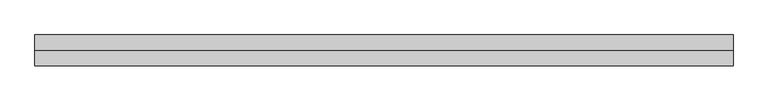
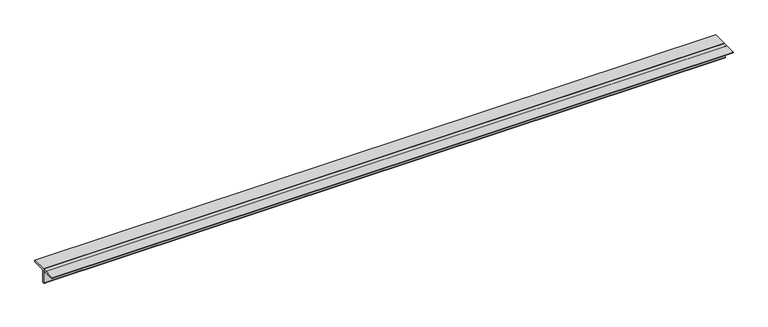
"""IFC4 building model written with IfcOpenShell, lengths in millimetres: member geometry, Steel Framing_2Ls_KS : H_SB_AR_S02_2Ls-100x100x10_VBR1."""

from ifc_helpers import new_model, si_unit, point, frame, frame_2d, origin, place, context, project, spatial, polyline, circle_curve, trimmed, segment, composite_curve, outline, extrude, source, transform, mapped, element, save


def member_d81a11a3(model_context):
    return source(origin(), model_context, "Body", "SweptSolid", [
        extrude(outline(composite_curve([segment(polyline([(0.0, 28.2), (100.0, 28.2)]), True, "CONTINUOUS"), segment(trimmed(circle_curve(frame_2d((90.0, 28.2)), 10.0), [point((100.0, 28.2))], [point((90.0, 18.2))], False, "CARTESIAN"), True, "CONTINUOUS"), segment(polyline([(90.0, 18.2), (20.0, 18.2)]), True, "CONTINUOUS"), segment(trimmed(circle_curve(frame_2d((20.0, 8.2)), 10.0), [point((20.0, 18.2))], [point((10.0, 8.2))], True, "CARTESIAN"), True, "CONTINUOUS"), segment(polyline([(10.0, 8.2), (10.0, -61.8)]), True, "CONTINUOUS"), segment(trimmed(circle_curve(frame_2d((0.0, -61.8)), 10.0), [point((10.0, -61.8))], [point((0.0, -71.8))], False, "CARTESIAN"), True, "CONTINUOUS"), segment(polyline([(0.0, -71.8), (0.0, 28.2)]), True, "CONTINUOUS")], self_intersect=False)), frame((-2072.1213123, 0.0, 0.0), z_axis=(1.0, 0.0, 0.0), x_axis=(0.0, 1.0, 0.0)), (0.0, 0.0, 1.0), 4551.278999),
        extrude(outline(composite_curve([segment(polyline([(0.0, 28.2), (0.0, -71.8)]), True, "CONTINUOUS"), segment(trimmed(circle_curve(frame_2d((0.0, -61.8)), 10.0), [point((0.0, -71.8))], [point((-10.0, -61.8))], False, "CARTESIAN"), True, "CONTINUOUS"), segment(polyline([(-10.0, -61.8), (-10.0, 8.2)]), True, "CONTINUOUS"), segment(trimmed(circle_curve(frame_2d((-20.0, 8.2)), 10.0), [point((-10.0, 8.2))], [point((-20.0, 18.2))], True, "CARTESIAN"), True, "CONTINUOUS"), segment(polyline([(-20.0, 18.2), (-90.0, 18.2)]), True, "CONTINUOUS"), segment(trimmed(circle_curve(frame_2d((-90.0, 28.2)), 10.0), [point((-90.0, 18.2))], [point((-100.0, 28.2))], False, "CARTESIAN"), True, "CONTINUOUS"), segment(polyline([(-100.0, 28.2), (0.0, 28.2)]), True, "CONTINUOUS")], self_intersect=False)), frame((-2072.1213123, 0.0, 0.0), z_axis=(1.0, 0.0, 0.0), x_axis=(0.0, 1.0, 0.0)), (0.0, 0.0, 1.0), 4551.278999),
    ])


if __name__ == "__main__":
    model = new_model("IFC4")
    model_context = context("Model", 3, world=origin())
    ifc_project = project(units=[si_unit("LENGTHUNIT", "METRE", prefix="MILLI")], contexts=[model_context])
    site = spatial("IfcSite", under=ifc_project)
    building = spatial("IfcBuilding", under=site)
    placement = place(None, origin())
    member_shape = member_d81a11a3(model_context)
    element("IfcMember", 1, ObjectType="Steel Framing_2Ls_KS : H_SB_AR_S02_2Ls-100x100x10_VBR1", at=placement, inside=building, context=model_context, shape_type="MappedRepresentation", body=[
        mapped(member_shape, transform((0.0, 0.0, 0.0), x_axis=(1.0, 0.0, 0.0), y_axis=(0.0, 1.0, 0.0), z_axis=(0.0, 0.0, 1.0))),
    ])
    save(model, "model.ifc")

# Revit data of these elements
# Type "Steel Framing_2Ls_KS : H_SB_AR_S02_2Ls-100x100x10_VBR1"
#   Type Comments = "MAIN"
#   Type Mark = "VBR1"
#   H_SectionID = "2Ls-100x100x10"
#   Assembly Code = "B10"
#   Legs = "LLBB"
#   H_Ratio for Additional Steel Plate = 0.2
#   W = 0
#   Perimeter = 0.80 m²/m
#   Nominal Weight = 29.80 kgf/m
#   Length [instance default] = 1524 mm
#   Space = 0 mm
#   b = 100 mm
#   d = 100 mm
#   t = 10 mm
#   y = 28.2 mm
#   A = 0.0038 m²
#   Structural Material [instance default] = Steel, 45-345
# Element 1 (IfcMember, "Steel Framing_2Ls_KS : H_SB_AR_S02_2Ls-100x100x10_VBR1")
#   Materials on its faces: "Steel, 45-345"
# Materials
#   "Steel, 45-345": class "Metal", colour RGB 189 187 185, transparency 0, Description = "Steel 345 MPa", Cost = 0
